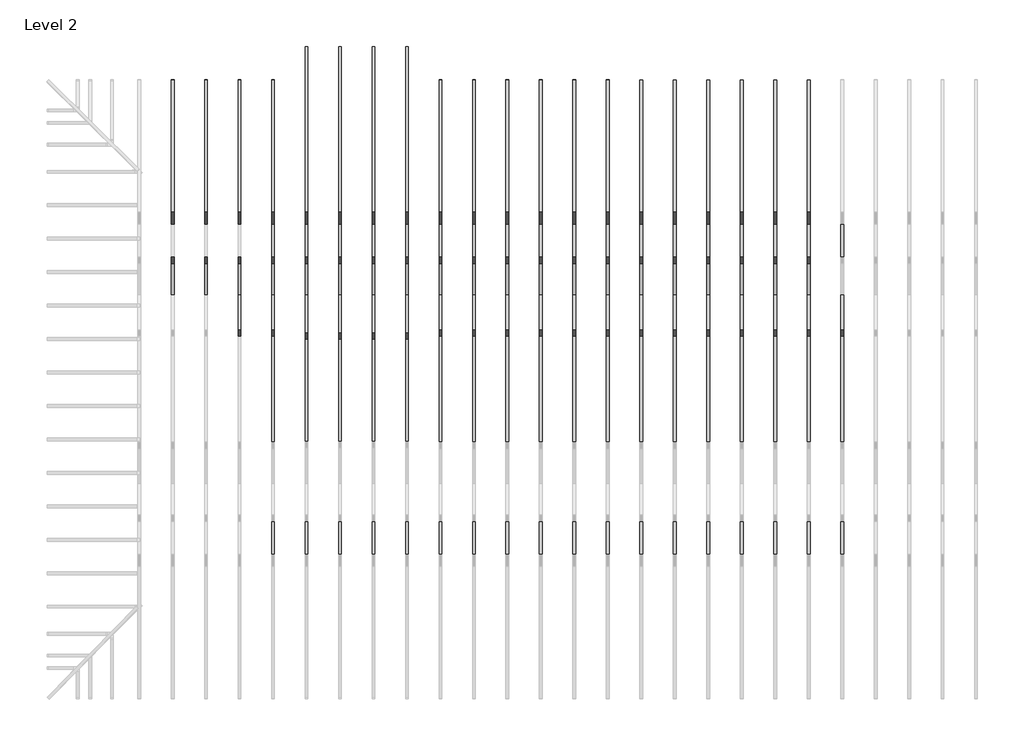
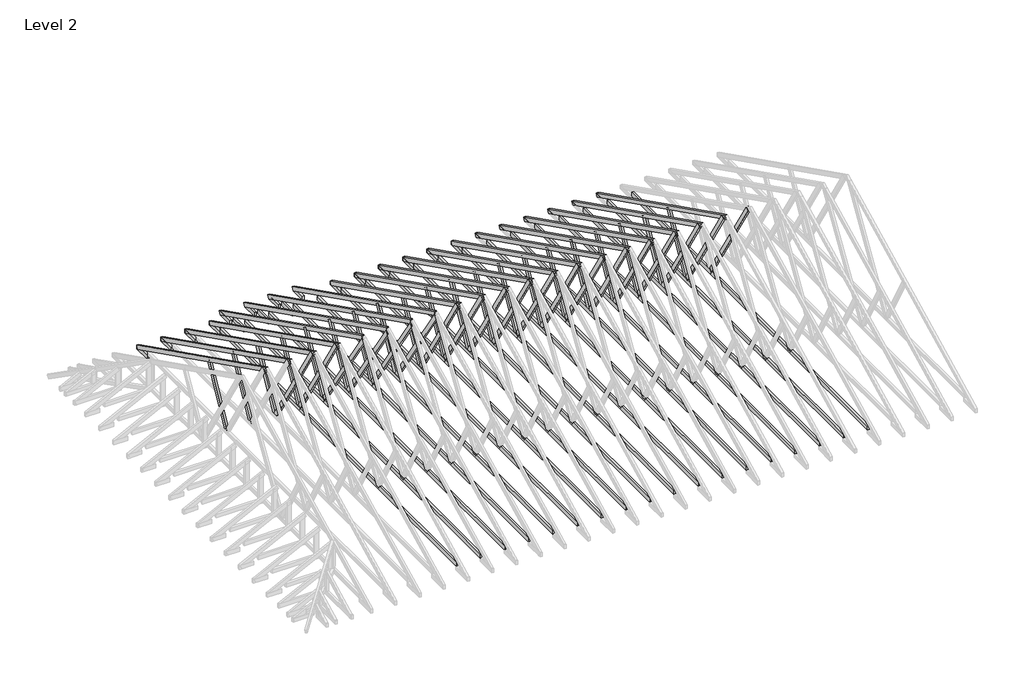
# One storey, part 4 of 5: 96 beams.
"""IFC4 building model written with IfcOpenShell, lengths in millimetres."""

import ifcopenshell
import ifcopenshell.guid

model = None  # the IFC model being written
_history = None  # IfcOwnerHistory: only IFC2X3 demands one
_inside = {}  # id of a spatial element -> (the spatial element, [elements in it])
_under = {}  # id of a project, library or spatial element -> (it, [spatial elements below it])
_declared = {}  # id of a project -> (the project, [libraries it declares])
_typed = {}  # id of a type object -> (the type object, [elements of that type])
_made_of = {}  # id of a material, layer set ... -> (it, [elements and type objects made of it])


def new_model(schema):
    """Start an empty IFC model of exactly this schema.

    Asked for "IFC4X3", IfcOpenShell would pick the latest addendum, in which some entities
    have other attributes; the version numbers below select the first issue.
    IFC2X3 requires an IfcOwnerHistory on every rooted entity: one is made here for all.
    """
    global model, _history
    if schema == "IFC4X3":
        model = ifcopenshell.file(schema_version=(4, 3, 0, 0))
    else:
        model = ifcopenshell.file(schema=schema)
    _inside.clear()
    _under.clear()
    _declared.clear()
    _typed.clear()
    _made_of.clear()
    _history = None
    if model.schema == "IFC2X3":
        org = make("IfcOrganization", Name="unknown")
        user = make(
            "IfcPersonAndOrganization",
            ThePerson=make("IfcPerson", FamilyName="unknown"),
            TheOrganization=org,
        )
        app = make(
            "IfcApplication",
            ApplicationDeveloper=org,
            Version="unknown",
            ApplicationFullName="unknown",
            ApplicationIdentifier="unknown",
        )
        _history = make(
            "IfcOwnerHistory",
            OwningUser=user,
            OwningApplication=app,
            ChangeAction="ADDED",
            CreationDate=0,
        )
    return model


def make(cls, **values):
    """One entity of the class cls with the attributes given. An attribute that is None is left unset."""
    return model.create_entity(
        cls, **{name: value for name, value in values.items() if value is not None}
    )


def rooted(cls, **values):
    """An entity with a GlobalId (a new one), such as an element, a storey or a relation."""
    return make(cls, GlobalId=ifcopenshell.guid.new(), OwnerHistory=_history, **values)


def si_unit(unit_type, name, prefix=None):
    """IfcSIUnit, for example si_unit("LENGTHUNIT", "METRE", prefix="MILLI")."""
    return make("IfcSIUnit", UnitType=unit_type, Prefix=prefix, Name=name)


def assignment(units):
    """IfcUnitAssignment: the units of a project."""
    return None if units is None else make("IfcUnitAssignment", Units=units)


def point(xyz):
    """IfcCartesianPoint."""
    return None if xyz is None else make("IfcCartesianPoint", Coordinates=xyz)


def direction(xyz):
    """IfcDirection."""
    return None if xyz is None else make("IfcDirection", DirectionRatios=xyz)


def frame(location, z_axis=None, x_axis=None):
    """IfcAxis2Placement3D, a coordinate frame: its origin and axes. An axis left out is left unset."""
    return make(
        "IfcAxis2Placement3D",
        Location=point(location),
        Axis=direction(z_axis),
        RefDirection=direction(x_axis),
    )


def origin():
    """The frame at (0, 0, 0) with its axes left unset."""
    return frame((0.0, 0.0, 0.0))


def place(relative_to, where):
    """IfcLocalPlacement: puts the frame where relative to a parent placement (None: the world)."""
    return make(
        "IfcLocalPlacement", PlacementRelTo=relative_to, RelativePlacement=where
    )


def context(
    kind, dimensions, precision=None, world=None, true_north=None, identifier=None
):
    """IfcGeometricRepresentationContext, for example the 3D "Model" context."""
    return make(
        "IfcGeometricRepresentationContext",
        ContextIdentifier=identifier,
        ContextType=kind,
        CoordinateSpaceDimension=dimensions,
        Precision=precision,
        WorldCoordinateSystem=world,
        TrueNorth=true_north,
    )


def project(units=None, contexts=None):
    """IfcProject with its units and contexts."""
    return rooted(
        "IfcProject",
        Name="project",
        RepresentationContexts=contexts,
        UnitsInContext=assignment(units),
    )


def spatial(cls, under=None, at=None, **own):
    """A site, building, storey or space (cls), placed at a placement, below another one or the project."""
    s = rooted(cls, ObjectPlacement=at, **own)
    if under is not None:
        _under.setdefault(under.id(), (under, []))[1].append(s)
    return s


def polyline(points):
    """IfcPolyline through the points."""
    return make("IfcPolyline", Points=[point(p) for p in points])


def outline(outer, holes=None, kind="AREA"):
    """IfcArbitraryClosedProfileDef: a profile drawn as a closed curve; with holes, ...WithVoids."""
    if holes is None:
        return make("IfcArbitraryClosedProfileDef", ProfileType=kind, OuterCurve=outer)
    return make(
        "IfcArbitraryProfileDefWithVoids",
        ProfileType=kind,
        OuterCurve=outer,
        InnerCurves=holes,
    )


def extrude(swept, where, along, depth):
    """IfcExtrudedAreaSolid: the profile swept, set in the frame where, extruded along a direction by depth."""
    return make(
        "IfcExtrudedAreaSolid",
        SweptArea=swept,
        Position=where,
        ExtrudedDirection=direction(along),
        Depth=depth,
    )


def shape(context_of_items, identifier, shape_type, items):
    """IfcShapeRepresentation: the items that make up one representation, for example the "Body"."""
    return make(
        "IfcShapeRepresentation",
        ContextOfItems=context_of_items,
        RepresentationIdentifier=identifier,
        RepresentationType=shape_type,
        Items=items,
    )


def source(mapping_origin, context_of_items, identifier, shape_type, items):
    """IfcRepresentationMap: a shape defined once, which mapped items show again and again."""
    return make(
        "IfcRepresentationMap",
        MappingOrigin=mapping_origin,
        MappedRepresentation=shape(context_of_items, identifier, shape_type, items),
    )


def transform(
    local_origin,
    x_axis=None,
    y_axis=None,
    z_axis=None,
    scale=None,
    scale2=None,
    scale3=None,
    uniform=True,
):
    """IfcCartesianTransformationOperator3D, or its non-uniform kind. x_axis, y_axis, z_axis: its Axis1, 2, 3."""
    if uniform:
        return make(
            "IfcCartesianTransformationOperator3D",
            Axis1=direction(x_axis),
            Axis2=direction(y_axis),
            LocalOrigin=point(local_origin),
            Scale=scale,
            Axis3=direction(z_axis),
        )
    return make(
        "IfcCartesianTransformationOperator3DnonUniform",
        Axis1=direction(x_axis),
        Axis2=direction(y_axis),
        LocalOrigin=point(local_origin),
        Scale=scale,
        Axis3=direction(z_axis),
        Scale2=scale2,
        Scale3=scale3,
    )


def mapped(mapping_source, mapping_target):
    """IfcMappedItem: shows the shape of a source again, moved by a transform."""
    return make(
        "IfcMappedItem", MappingSource=mapping_source, MappingTarget=mapping_target
    )


def made_of(thing, what):
    """Note that an element or type object is made of a material, layer set ...; save() writes the relation."""
    if what is not None:
        _made_of.setdefault(what.id(), (what, []))[1].append(thing)
    return thing


def element(
    cls,
    number,
    at=None,
    inside=None,
    cuts=None,
    type_object=None,
    material=None,
    context=None,
    identifier="Body",
    shape_type=None,
    held_by="IfcProductDefinitionShape",
    body=None,
    shapes=None,
    **own,
):
    """One element of the class cls, such as IfcWall. Its Tag is "e" and its number.

    at: its placement. inside: the storey or other place that contains it. cuts: it is an
    opening in that element (IfcRelVoidsElement). A single representation is given by context,
    identifier, shape_type and body (its items); several are given by shapes. held_by: the class
    of the entity that holds the representations. save() writes the other relations.
    """
    e = rooted(cls, Tag="e%d" % number, ObjectPlacement=at, **own)
    if body is not None:
        shapes = [shape(context, identifier, shape_type, body)]
    if shapes is not None:
        e.Representation = make(held_by, Representations=shapes)
    if inside is not None:
        _inside.setdefault(inside.id(), (inside, []))[1].append(e)
    if cuts is not None:
        rooted(
            "IfcRelVoidsElement", RelatingBuildingElement=cuts, RelatedOpeningElement=e
        )
    if type_object is not None:
        _typed.setdefault(type_object.id(), (type_object, []))[1].append(e)
    return made_of(e, material)


def aggregate(whole, parts):
    """IfcRelAggregates: a whole, such as a stair, and the parts it consists of."""
    return rooted("IfcRelAggregates", RelatingObject=whole, RelatedObjects=parts)


def save(model, path):
    """Write the relations noted so far, then the file.

    IfcRelAggregates (storeys below a building ...), IfcRelContainedInSpatialStructure (elements
    in a storey), IfcRelDefinesByType, IfcRelAssociatesMaterial and IfcRelDeclares: one each for
    every whole, place, type object, material and project.
    """
    for whole, parts in _under.values():
        aggregate(whole, parts)
    for where, things in _inside.values():
        rooted(
            "IfcRelContainedInSpatialStructure",
            RelatedElements=things,
            RelatingStructure=where,
        )
    for kind, things in _typed.values():
        rooted("IfcRelDefinesByType", RelatedObjects=things, RelatingType=kind)
    for what, things in _made_of.values():
        rooted("IfcRelAssociatesMaterial", RelatedObjects=things, RelatingMaterial=what)
    for by, libraries in _declared.values():
        rooted("IfcRelDeclares", RelatingContext=by, RelatedDefinitions=libraries)
    model.write(path)


def beam_b78a0881(model_context):
    return source(origin(), model_context, "Body", "SweptSolid", [
        extrude(outline(polyline([(228.6, 25.4), (228.6, -25.4), (-228.6, -25.4), (-228.6, 25.4), (228.6, 25.4)])), frame((0.0, 0.0, -50.8), z_axis=(0.0, 0.0, 1.0), x_axis=(1.0, 0.0, 0.0)), (0.0, 0.0, 1.0), 101.6),
    ])


def beam_90eea034(model_context):
    return source(origin(), model_context, "Body", "SweptSolid", [
        extrude(outline(polyline([(821.193698, 25.4), (821.193698, -25.4), (-819.5010489, -25.4), (-819.5010489, 25.4), (821.193698, 25.4)])), frame((0.0, 0.0, -50.8), z_axis=(0.0, 0.0, 1.0), x_axis=(1.0, 0.0, 0.0)), (0.0, 0.0, 1.0), 101.6),
    ])


def beam_a4242642(model_context):
    return source(origin(), model_context, "Body", "SweptSolid", [
        extrude(outline(polyline([(5145.3336481, 25.4), (5145.3336481, -25.4), (-5145.3336481, -25.4), (-5145.3336481, 25.4), (5145.3336481, 25.4)])), frame((0.0, 0.0, -50.8), z_axis=(0.0, 0.0, 1.0), x_axis=(1.0, 0.0, 0.0)), (0.0, 0.0, 1.0), 101.6),
    ])


def beam_fc8bf4ae(model_context):
    return source(origin(), model_context, "Body", "SweptSolid", [
        extrude(outline(polyline([(1562.6646551, 25.4), (1562.6646551, -25.4), (-1550.1468127, -25.4), (-1550.1468127, 25.4), (1562.6646551, 25.4)])), frame((0.0, 0.0, -50.8), z_axis=(0.0, 0.0, 1.0), x_axis=(1.0, 0.0, 0.0)), (0.0, 0.0, 1.0), 101.6),
    ])


def beam_2924e986(model_context):
    return source(origin(), model_context, "Body", "SweptSolid", [
        extrude(outline(polyline([(228.5999994, 25.4), (228.5999994, -25.4), (-179.8629717, -25.4), (-179.8629717, 25.4), (228.5999994, 25.4)])), frame((0.0, 0.0, -50.8), z_axis=(0.0, 0.0, 1.0), x_axis=(1.0, 0.0, 0.0)), (0.0, 0.0, 1.0), 101.6),
    ])


def beam_189f326c(model_context):
    return source(origin(), model_context, "Body", "SweptSolid", [
        extrude(outline(polyline([(1574.4380265, 25.4), (1574.4380265, -25.4), (-1601.4606477, -25.4), (-1601.4606477, 25.4), (1574.4380265, 25.4)])), frame((0.0, 0.0, -50.8), z_axis=(0.0, 0.0, 1.0), x_axis=(1.0, 0.0, 0.0)), (0.0, 0.0, 1.0), 101.6),
    ])


def beam_af7bd0b6(model_context):
    return source(origin(), model_context, "Body", "SweptSolid", [
        extrude(outline(polyline([(228.6, 25.4), (228.6, -25.4), (-179.8629717, -25.4), (-179.8629717, 25.4), (228.6, 25.4)])), frame((0.0, 0.0, -50.8), z_axis=(0.0, 0.0, 1.0), x_axis=(1.0, 0.0, 0.0)), (0.0, 0.0, 1.0), 101.6),
    ])


model = new_model("IFC4")

# Units and contexts
model_context = context("Model", 3, world=origin())
ifc_project = project(units=[si_unit("LENGTHUNIT", "METRE", prefix="MILLI")], contexts=[model_context])

# Site, building, storey
site = spatial("IfcSite", under=ifc_project)
building = spatial("IfcBuilding", under=site)
storey = spatial("IfcBuildingStorey", under=building, Name="Level 2", Elevation=2768.6)

# Beams
placement = place(None, origin())
element("IfcBeam", 1, ObjectType="Dimension Lumber : BLDG 6241 2X4\" TRUSS MEMBER", at=placement, inside=storey, context=model_context, shape_type="SweptSolid", body=[
    extrude(outline(polyline([(0.0, -50.8), (0.0, 0.0), (6948.260151, 0.0), (6948.260151, -50.8), (0.0, -50.8)])), frame((-13559.414829, 10.7781069, 5482.082899), z_axis=(0.0, 0.4472135954999579, 0.894427190999916), x_axis=(0.0, 0.894427190999916, -0.4472135954999579)), (0.0, 0.0, 1.0), 101.6),
])
element("IfcBeam", 2, ObjectType="Dimension Lumber : BLDG 6241 2X4\" TRUSS MEMBER", at=placement, inside=storey, context=model_context, shape_type="SweptSolid", body=[
    extrude(outline(polyline([(0.0, -50.8), (0.0, 0.0), (6948.260151, 0.0), (6948.260151, -50.8), (0.0, -50.8)])), frame((-12949.814829, 10.7781069, 5482.082899), z_axis=(0.0, 0.44721359549995804, 0.894427190999916), x_axis=(0.0, 0.894427190999916, -0.44721359549995804)), (0.0, 0.0, 1.0), 101.6),
])
element("IfcBeam", 3, ObjectType="Dimension Lumber : BLDG 6241 2X4\" TRUSS MEMBER", at=placement, inside=storey, context=model_context, shape_type="SweptSolid", body=[
    extrude(outline(polyline([(0.0, -50.8), (0.0, 0.0), (6948.260151, 0.0), (6948.260151, -50.8), (0.0, -50.8)])), frame((-12340.214829, 10.7781069, 5482.082899), z_axis=(0.0, 0.44721359549995804, 0.894427190999916), x_axis=(0.0, 0.894427190999916, -0.44721359549995804)), (0.0, 0.0, 1.0), 101.6),
])
element("IfcBeam", 4, ObjectType="Dimension Lumber : BLDG 6241 2X4\" TRUSS MEMBER", at=placement, inside=storey, context=model_context, shape_type="SweptSolid", body=[
    extrude(outline(polyline([(0.0, -50.8), (0.0, 0.0), (6948.260151, 0.0), (6948.260151, -50.8), (0.0, -50.8)])), frame((-11730.614829, 10.7781069, 5482.082899), z_axis=(0.0, 0.44721359549995804, 0.894427190999916), x_axis=(0.0, 0.894427190999916, -0.44721359549995804)), (0.0, 0.0, 1.0), 101.6),
])
element("IfcBeam", 5, ObjectType="Dimension Lumber : BLDG 6241 2X4\" TRUSS MEMBER", at=placement, inside=storey, context=model_context, shape_type="SweptSolid", body=[
    extrude(outline(polyline([(0.0, -50.8), (0.0, 0.0), (6302.2496334, 0.0), (6302.2496334, -50.8), (0.0, -50.8)])), frame((-15997.814829, -17.2791662, 5496.1115355), z_axis=(0.0, 0.447213595499956, 0.894427190999917), x_axis=(0.0, 0.894427190999917, -0.447213595499956)), (0.0, 0.0, 1.0), 101.6),
])
element("IfcBeam", 6, ObjectType="Dimension Lumber : BLDG 6241 2X4\" TRUSS MEMBER", at=placement, inside=storey, context=model_context, shape_type="SweptSolid", body=[
    extrude(outline(polyline([(0.0, -50.8), (0.0, 0.0), (6302.2496334, 0.0), (6302.2496334, -50.8), (0.0, -50.8)])), frame((-15388.214829, -17.2791662, 5496.1115355), z_axis=(0.0, 0.447213595499956, 0.894427190999917), x_axis=(0.0, 0.894427190999917, -0.447213595499956)), (0.0, 0.0, 1.0), 101.6),
])
element("IfcBeam", 7, ObjectType="Dimension Lumber : BLDG 6241 2X4\" TRUSS MEMBER", at=placement, inside=storey, context=model_context, shape_type="SweptSolid", body=[
    extrude(outline(polyline([(0.0, -50.8), (0.0, 0.0), (6302.2496334, 0.0), (6302.2496334, -50.8), (0.0, -50.8)])), frame((-14778.614829, -17.2791662, 5496.1115355), z_axis=(0.0, 0.44721359549995576, 0.8944271909999171), x_axis=(0.0, 0.8944271909999171, -0.44721359549995576)), (0.0, 0.0, 1.0), 101.6),
])
element("IfcBeam", 8, ObjectType="Dimension Lumber : BLDG 6241 2X4\" TRUSS MEMBER", at=placement, inside=storey, context=model_context, shape_type="SweptSolid", body=[
    extrude(outline(polyline([(0.0, -50.8), (0.0, 0.0), (6302.2496334, 0.0), (6302.2496334, -50.8), (0.0, -50.8)])), frame((-14169.014829, -17.2791662, 5496.1115355), z_axis=(0.0, 0.447213595499956, 0.894427190999917), x_axis=(0.0, 0.894427190999917, -0.447213595499956)), (0.0, 0.0, 1.0), 101.6),
])
element("IfcBeam", 9, ObjectType="Dimension Lumber : BLDG 6241 2X4\" TRUSS MEMBER", at=placement, inside=storey, context=model_context, shape_type="SweptSolid", body=[
    extrude(outline(polyline([(0.0, -50.8), (0.0, 0.0), (6302.2496334, 0.0), (6302.2496334, -50.8), (0.0, -50.8)])), frame((-11121.014829, -17.2791662, 5496.1115355), z_axis=(0.0, 0.447213595499956, 0.894427190999917), x_axis=(0.0, 0.894427190999917, -0.447213595499956)), (0.0, 0.0, 1.0), 101.6),
])
element("IfcBeam", 10, ObjectType="Dimension Lumber : BLDG 6241 2X4\" TRUSS MEMBER", at=placement, inside=storey, context=model_context, shape_type="SweptSolid", body=[
    extrude(outline(polyline([(0.0, -50.8), (0.0, 0.0), (6302.2496334, 0.0), (6302.2496334, -50.8), (0.0, -50.8)])), frame((-10511.414829, -17.2791662, 5496.1115355), z_axis=(0.0, 0.4472135954999559, 0.894427190999917), x_axis=(0.0, 0.894427190999917, -0.4472135954999559)), (0.0, 0.0, 1.0), 101.6),
])
element("IfcBeam", 11, ObjectType="Dimension Lumber : BLDG 6241 2X4\" TRUSS MEMBER", at=placement, inside=storey, context=model_context, shape_type="SweptSolid", body=[
    extrude(outline(polyline([(0.0, -50.8), (0.0, 0.0), (6302.2496334, 0.0), (6302.2496334, -50.8), (0.0, -50.8)])), frame((-9901.814829, -17.2791662, 5496.1115355), z_axis=(0.0, 0.44721359549995576, 0.894427190999917), x_axis=(0.0, 0.894427190999917, -0.44721359549995576)), (0.0, 0.0, 1.0), 101.6),
])
element("IfcBeam", 12, ObjectType="Dimension Lumber : BLDG 6241 2X4\" TRUSS MEMBER", at=placement, inside=storey, context=model_context, shape_type="SweptSolid", body=[
    extrude(outline(polyline([(0.0, -50.8), (0.0, 0.0), (6302.2496334, 0.0), (6302.2496334, -50.8), (0.0, -50.8)])), frame((-9292.214829, -17.2791662, 5496.1115355), z_axis=(0.0, 0.447213595499956, 0.8944271909999169), x_axis=(0.0, 0.8944271909999169, -0.447213595499956)), (0.0, 0.0, 1.0), 101.6),
])
element("IfcBeam", 13, ObjectType="Dimension Lumber : BLDG 6241 2X4\" TRUSS MEMBER", at=placement, inside=storey, context=model_context, shape_type="SweptSolid", body=[
    extrude(outline(polyline([(0.0, -50.8), (0.0, 0.0), (6302.2496334, 0.0), (6302.2496334, -50.8), (0.0, -50.8)])), frame((-8682.614829, -17.2791662, 5496.1115355), z_axis=(0.0, 0.44721359549995593, 0.894427190999917), x_axis=(0.0, 0.894427190999917, -0.44721359549995593)), (0.0, 0.0, 1.0), 101.6),
])
element("IfcBeam", 14, ObjectType="Dimension Lumber : BLDG 6241 2X4\" TRUSS MEMBER", at=placement, inside=storey, context=model_context, shape_type="SweptSolid", body=[
    extrude(outline(polyline([(0.0, -50.8), (0.0, 0.0), (6302.2496334, 0.0), (6302.2496334, -50.8), (0.0, -50.8)])), frame((-8073.014829, -17.2791662, 5496.1115355), z_axis=(0.0, 0.4472135954999558, 0.894427190999917), x_axis=(0.0, 0.894427190999917, -0.4472135954999558)), (0.0, 0.0, 1.0), 101.6),
])
element("IfcBeam", 15, ObjectType="Dimension Lumber : BLDG 6241 2X4\" TRUSS MEMBER", at=placement, inside=storey, context=model_context, shape_type="SweptSolid", body=[
    extrude(outline(polyline([(0.0, -50.8), (0.0, 0.0), (6302.2496334, 0.0), (6302.2496334, -50.8), (0.0, -50.8)])), frame((-7463.414829, -17.2791662, 5496.1115355), z_axis=(0.0, 0.4472135954999557, 0.894427190999917), x_axis=(0.0, 0.894427190999917, -0.4472135954999557)), (0.0, 0.0, 1.0), 101.6),
])
element("IfcBeam", 16, ObjectType="Dimension Lumber : BLDG 6241 2X4\" TRUSS MEMBER", at=placement, inside=storey, context=model_context, shape_type="SweptSolid", body=[
    extrude(outline(polyline([(0.0, -50.8), (0.0, 0.0), (6302.2496334, 0.0), (6302.2496334, -50.8), (0.0, -50.8)])), frame((-6853.814829, -17.2791662, 5496.1115355), z_axis=(0.0, 0.4472135954999561, 0.8944271909999169), x_axis=(0.0, 0.8944271909999169, -0.4472135954999561)), (0.0, 0.0, 1.0), 101.6),
])
element("IfcBeam", 17, ObjectType="Dimension Lumber : BLDG 6241 2X4\" TRUSS MEMBER", at=placement, inside=storey, context=model_context, shape_type="SweptSolid", body=[
    extrude(outline(polyline([(0.0, -50.8), (0.0, 0.0), (6302.2496334, 0.0), (6302.2496334, -50.8), (0.0, -50.8)])), frame((-6244.214829, -17.2791662, 5496.1115355), z_axis=(0.0, 0.44721359549995593, 0.894427190999917), x_axis=(0.0, 0.894427190999917, -0.44721359549995593)), (0.0, 0.0, 1.0), 101.6),
])
element("IfcBeam", 18, ObjectType="Dimension Lumber : BLDG 6241 2X4\" TRUSS MEMBER", at=placement, inside=storey, context=model_context, shape_type="SweptSolid", body=[
    extrude(outline(polyline([(0.0, -50.8), (0.0, 0.0), (6302.2496334, 0.0), (6302.2496334, -50.8), (0.0, -50.8)])), frame((-5634.614829, -17.2791662, 5496.1115355), z_axis=(0.0, 0.447213595499956, 0.8944271909999169), x_axis=(0.0, 0.8944271909999169, -0.447213595499956)), (0.0, 0.0, 1.0), 101.6),
])
element("IfcBeam", 19, ObjectType="Dimension Lumber : BLDG 6241 2X4\" TRUSS MEMBER", at=placement, inside=storey, context=model_context, shape_type="SweptSolid", body=[
    extrude(outline(polyline([(0.0, -50.8), (0.0, 0.0), (6302.2496334, 0.0), (6302.2496334, -50.8), (0.0, -50.8)])), frame((-5025.014829, -17.2791662, 5496.1115355), z_axis=(0.0, 0.44721359549995593, 0.894427190999917), x_axis=(0.0, 0.894427190999917, -0.44721359549995593)), (0.0, 0.0, 1.0), 101.6),
])
element("IfcBeam", 20, ObjectType="Dimension Lumber : BLDG 6241 2X4\" TRUSS MEMBER", at=placement, inside=storey, context=model_context, shape_type="SweptSolid", body=[
    extrude(outline(polyline([(0.0, -50.8), (0.0, 0.0), (6302.2496334, 0.0), (6302.2496334, -50.8), (0.0, -50.8)])), frame((-4415.414829, -17.2791662, 5496.1115355), z_axis=(0.0, 0.4472135954999558, 0.894427190999917), x_axis=(0.0, 0.894427190999917, -0.4472135954999558)), (0.0, 0.0, 1.0), 101.6),
])
beam_shape = beam_b78a0881(model_context)
element("IfcBeam", 21, ObjectType="Dimension Lumber : BLDG 6241 2X4\" TRUSS MEMBER", at=placement, inside=storey, context=model_context, shape_type="MappedRepresentation", body=[
    mapped(beam_shape, transform((-13534.014829, 5436.3284114, 2589.5072623), x_axis=(0.0, -1.0, 0.0), y_axis=(1.0, 0.0, 0.0), z_axis=(0.0, 0.0, 1.0))),
])
element("IfcBeam", 22, ObjectType="Dimension Lumber : BLDG 6241 2X4\" TRUSS MEMBER", at=placement, inside=storey, context=model_context, shape_type="MappedRepresentation", body=[
    mapped(beam_shape, transform((-12924.414829, 5436.3284114, 2589.5072623), x_axis=(0.0, -1.0, 0.0), y_axis=(1.0, 0.0, 0.0), z_axis=(0.0, 0.0, 1.0))),
])
element("IfcBeam", 23, ObjectType="Dimension Lumber : BLDG 6241 2X4\" TRUSS MEMBER", at=placement, inside=storey, context=model_context, shape_type="MappedRepresentation", body=[
    mapped(beam_shape, transform((-12314.814829, 5436.3284114, 2589.5072623), x_axis=(0.0, -1.0, 0.0), y_axis=(1.0, 0.0, 0.0), z_axis=(0.0, 0.0, 1.0))),
])
element("IfcBeam", 24, ObjectType="Dimension Lumber : BLDG 6241 2X4\" TRUSS MEMBER", at=placement, inside=storey, context=model_context, shape_type="MappedRepresentation", body=[
    mapped(beam_shape, transform((-12924.414829, 5436.3284114, 2589.5072623), x_axis=(0.0, -1.0, 0.0), y_axis=(1.0, 0.0, 0.0), z_axis=(0.0, 0.0, 1.0))),
])
element("IfcBeam", 25, ObjectType="Dimension Lumber : BLDG 6241 2X4\" TRUSS MEMBER", at=placement, inside=storey, context=model_context, shape_type="MappedRepresentation", body=[
    mapped(beam_shape, transform((-12314.814829, 5436.3284114, 2589.5072623), x_axis=(0.0, -1.0, 0.0), y_axis=(1.0, 0.0, 0.0), z_axis=(0.0, 0.0, 1.0))),
])
element("IfcBeam", 26, ObjectType="Dimension Lumber : BLDG 6241 2X4\" TRUSS MEMBER", at=placement, inside=storey, context=model_context, shape_type="MappedRepresentation", body=[
    mapped(beam_shape, transform((-15972.414829, 5436.3284114, 2717.8), x_axis=(0.0, -1.0, 0.0), y_axis=(1.0, 0.0, 0.0), z_axis=(0.0, 0.0, 1.0))),
])
element("IfcBeam", 27, ObjectType="Dimension Lumber : BLDG 6241 2X4\" TRUSS MEMBER", at=placement, inside=storey, context=model_context, shape_type="MappedRepresentation", body=[
    mapped(beam_shape, transform((-15362.814829, 5436.3284114, 2717.8), x_axis=(0.0, -1.0, 0.0), y_axis=(1.0, 0.0, 0.0), z_axis=(0.0, 0.0, 1.0))),
])
element("IfcBeam", 28, ObjectType="Dimension Lumber : BLDG 6241 2X4\" TRUSS MEMBER", at=placement, inside=storey, context=model_context, shape_type="MappedRepresentation", body=[
    mapped(beam_shape, transform((-14753.214829, 5436.3284114, 2717.8), x_axis=(0.0, -1.0, 0.0), y_axis=(1.0, 0.0, 0.0), z_axis=(0.0, 0.0, 1.0))),
])
element("IfcBeam", 29, ObjectType="Dimension Lumber : BLDG 6241 2X4\" TRUSS MEMBER", at=placement, inside=storey, context=model_context, shape_type="MappedRepresentation", body=[
    mapped(beam_shape, transform((-14143.614829, 5436.3284114, 2717.8), x_axis=(0.0, -1.0, 0.0), y_axis=(1.0, 0.0, 0.0), z_axis=(0.0, 0.0, 1.0))),
])
element("IfcBeam", 30, ObjectType="Dimension Lumber : BLDG 6241 2X4\" TRUSS MEMBER", at=placement, inside=storey, context=model_context, shape_type="MappedRepresentation", body=[
    mapped(beam_shape, transform((-11095.614829, 5436.3284114, 2717.8), x_axis=(0.0, -1.0, 0.0), y_axis=(1.0, 0.0, 0.0), z_axis=(0.0, 0.0, 1.0))),
])
element("IfcBeam", 31, ObjectType="Dimension Lumber : BLDG 6241 2X4\" TRUSS MEMBER", at=placement, inside=storey, context=model_context, shape_type="MappedRepresentation", body=[
    mapped(beam_shape, transform((-10486.014829, 5436.3284114, 2717.8), x_axis=(0.0, -1.0, 0.0), y_axis=(1.0, 0.0, 0.0), z_axis=(0.0, 0.0, 1.0))),
])
element("IfcBeam", 32, ObjectType="Dimension Lumber : BLDG 6241 2X4\" TRUSS MEMBER", at=placement, inside=storey, context=model_context, shape_type="MappedRepresentation", body=[
    mapped(beam_shape, transform((-9876.414829, 5436.3284114, 2717.8), x_axis=(0.0, -1.0, 0.0), y_axis=(1.0, 0.0, 0.0), z_axis=(0.0, 0.0, 1.0))),
])
element("IfcBeam", 33, ObjectType="Dimension Lumber : BLDG 6241 2X4\" TRUSS MEMBER", at=placement, inside=storey, context=model_context, shape_type="MappedRepresentation", body=[
    mapped(beam_shape, transform((-9266.814829, 5436.3284114, 2717.8), x_axis=(0.0, -1.0, 0.0), y_axis=(1.0, 0.0, 0.0), z_axis=(0.0, 0.0, 1.0))),
])
element("IfcBeam", 34, ObjectType="Dimension Lumber : BLDG 6241 2X4\" TRUSS MEMBER", at=placement, inside=storey, context=model_context, shape_type="MappedRepresentation", body=[
    mapped(beam_shape, transform((-8657.214829, 5436.3284114, 2717.8), x_axis=(0.0, -1.0, 0.0), y_axis=(1.0, 0.0, 0.0), z_axis=(0.0, 0.0, 1.0))),
])
element("IfcBeam", 35, ObjectType="Dimension Lumber : BLDG 6241 2X4\" TRUSS MEMBER", at=placement, inside=storey, context=model_context, shape_type="MappedRepresentation", body=[
    mapped(beam_shape, transform((-8047.614829, 5436.3284114, 2717.8), x_axis=(0.0, -1.0, 0.0), y_axis=(1.0, 0.0, 0.0), z_axis=(0.0, 0.0, 1.0))),
])
beam_2_shape = beam_90eea034(model_context)
element("IfcBeam", 36, ObjectType="Dimension Lumber : BLDG 6241 2X4\" TRUSS MEMBER", at=placement, inside=storey, context=model_context, shape_type="MappedRepresentation", body=[
    mapped(beam_2_shape, transform((-13534.014829, 2147.8781861, 3552.5770493), x_axis=(0.0, -0.48031726308520883, -0.87709482200178), y_axis=(-1.0, 0.0, 0.0), z_axis=(0.0, 0.87709482200178, -0.48031726308520883))),
])
element("IfcBeam", 37, ObjectType="Dimension Lumber : BLDG 6241 2X4\" TRUSS MEMBER", at=placement, inside=storey, context=model_context, shape_type="MappedRepresentation", body=[
    mapped(beam_2_shape, transform((-12924.414829, 2147.8781861, 3552.5770493), x_axis=(0.0, -0.48031726308520883, -0.87709482200178), y_axis=(-1.0, 0.0, 0.0), z_axis=(0.0, 0.87709482200178, -0.48031726308520883))),
])
element("IfcBeam", 38, ObjectType="Dimension Lumber : BLDG 6241 2X4\" TRUSS MEMBER", at=placement, inside=storey, context=model_context, shape_type="MappedRepresentation", body=[
    mapped(beam_2_shape, transform((-12314.814829, 2147.8781861, 3552.5770493), x_axis=(0.0, -0.48031726308520883, -0.87709482200178), y_axis=(-1.0, 0.0, 0.0), z_axis=(0.0, 0.87709482200178, -0.48031726308520883))),
])
element("IfcBeam", 39, ObjectType="Dimension Lumber : BLDG 6241 2X4\" TRUSS MEMBER", at=placement, inside=storey, context=model_context, shape_type="MappedRepresentation", body=[
    mapped(beam_2_shape, transform((-11705.214829, 2147.8781861, 3552.5770493), x_axis=(0.0, -0.48031726308520883, -0.87709482200178), y_axis=(-1.0, 0.0, 0.0), z_axis=(0.0, 0.87709482200178, -0.48031726308520883))),
])
element("IfcBeam", 40, ObjectType="Dimension Lumber : BLDG 6241 2X4\" TRUSS MEMBER", at=placement, inside=storey, context=model_context, shape_type="MappedRepresentation", body=[
    mapped(beam_2_shape, transform((-15972.414829, 2147.8781861, 3552.5770493), x_axis=(0.0, -0.4803172630852004, -0.8770948220017847), y_axis=(-1.0, 0.0, 0.0), z_axis=(0.0, 0.8770948220017847, -0.4803172630852004))),
])
element("IfcBeam", 41, ObjectType="Dimension Lumber : BLDG 6241 2X4\" TRUSS MEMBER", at=placement, inside=storey, context=model_context, shape_type="MappedRepresentation", body=[
    mapped(beam_2_shape, transform((-15362.814829, 2147.8781861, 3552.5770493), x_axis=(0.0, -0.4803172630852004, -0.8770948220017847), y_axis=(-1.0, 0.0, 0.0), z_axis=(0.0, 0.8770948220017847, -0.4803172630852004))),
])
element("IfcBeam", 42, ObjectType="Dimension Lumber : BLDG 6241 2X4\" TRUSS MEMBER", at=placement, inside=storey, context=model_context, shape_type="MappedRepresentation", body=[
    mapped(beam_2_shape, transform((-14753.214829, 2147.8781861, 3552.5770493), x_axis=(0.0, -0.4803172630852004, -0.8770948220017847), y_axis=(-1.0, 0.0, 0.0), z_axis=(0.0, 0.8770948220017847, -0.4803172630852004))),
])
element("IfcBeam", 43, ObjectType="Dimension Lumber : BLDG 6241 2X4\" TRUSS MEMBER", at=placement, inside=storey, context=model_context, shape_type="MappedRepresentation", body=[
    mapped(beam_2_shape, transform((-14143.614829, 2147.8781861, 3552.5770493), x_axis=(0.0, -0.4803172630852004, -0.8770948220017847), y_axis=(-1.0, 0.0, 0.0), z_axis=(0.0, 0.8770948220017847, -0.4803172630852004))),
])
element("IfcBeam", 44, ObjectType="Dimension Lumber : BLDG 6241 2X4\" TRUSS MEMBER", at=placement, inside=storey, context=model_context, shape_type="MappedRepresentation", body=[
    mapped(beam_2_shape, transform((-11095.614829, 2147.8781861, 3552.5770493), x_axis=(0.0, -0.4803172630852004, -0.8770948220017847), y_axis=(-1.0, 0.0, 0.0), z_axis=(0.0, 0.8770948220017847, -0.4803172630852004))),
])
element("IfcBeam", 45, ObjectType="Dimension Lumber : BLDG 6241 2X4\" TRUSS MEMBER", at=placement, inside=storey, context=model_context, shape_type="MappedRepresentation", body=[
    mapped(beam_2_shape, transform((-10486.014829, 2147.8781861, 3552.5770493), x_axis=(0.0, -0.4803172630852004, -0.8770948220017847), y_axis=(-1.0, 0.0, 0.0), z_axis=(0.0, 0.8770948220017847, -0.4803172630852004))),
])
element("IfcBeam", 46, ObjectType="Dimension Lumber : BLDG 6241 2X4\" TRUSS MEMBER", at=placement, inside=storey, context=model_context, shape_type="MappedRepresentation", body=[
    mapped(beam_2_shape, transform((-9876.414829, 2147.8781861, 3552.5770493), x_axis=(0.0, -0.4803172630852004, -0.8770948220017847), y_axis=(-1.0, 0.0, 0.0), z_axis=(0.0, 0.8770948220017847, -0.4803172630852004))),
])
element("IfcBeam", 47, ObjectType="Dimension Lumber : BLDG 6241 2X4\" TRUSS MEMBER", at=placement, inside=storey, context=model_context, shape_type="MappedRepresentation", body=[
    mapped(beam_2_shape, transform((-9266.814829, 2147.8781861, 3552.5770493), x_axis=(0.0, -0.4803172630852004, -0.8770948220017847), y_axis=(-1.0, 0.0, 0.0), z_axis=(0.0, 0.8770948220017847, -0.4803172630852004))),
])
element("IfcBeam", 48, ObjectType="Dimension Lumber : BLDG 6241 2X4\" TRUSS MEMBER", at=placement, inside=storey, context=model_context, shape_type="MappedRepresentation", body=[
    mapped(beam_2_shape, transform((-8657.214829, 2147.8781861, 3552.5770493), x_axis=(0.0, -0.4803172630852004, -0.8770948220017847), y_axis=(-1.0, 0.0, 0.0), z_axis=(0.0, 0.8770948220017847, -0.4803172630852004))),
])
element("IfcBeam", 49, ObjectType="Dimension Lumber : BLDG 6241 2X4\" TRUSS MEMBER", at=placement, inside=storey, context=model_context, shape_type="MappedRepresentation", body=[
    mapped(beam_2_shape, transform((-8047.614829, 2147.8781861, 3552.5770493), x_axis=(0.0, -0.4803172630852004, -0.8770948220017847), y_axis=(-1.0, 0.0, 0.0), z_axis=(0.0, 0.8770948220017847, -0.4803172630852004))),
])
element("IfcBeam", 50, ObjectType="Dimension Lumber : BLDG 6241 2X4\" TRUSS MEMBER", at=placement, inside=storey, context=model_context, shape_type="MappedRepresentation", body=[
    mapped(beam_2_shape, transform((-7438.014829, 2147.8781861, 3552.5770493), x_axis=(0.0, -0.4803172630852004, -0.8770948220017847), y_axis=(-1.0, 0.0, 0.0), z_axis=(0.0, 0.8770948220017847, -0.4803172630852004))),
])
element("IfcBeam", 51, ObjectType="Dimension Lumber : BLDG 6241 2X4\" TRUSS MEMBER", at=placement, inside=storey, context=model_context, shape_type="MappedRepresentation", body=[
    mapped(beam_2_shape, transform((-6828.414829, 2147.8781861, 3552.5770493), x_axis=(0.0, -0.4803172630852004, -0.8770948220017847), y_axis=(-1.0, 0.0, 0.0), z_axis=(0.0, 0.8770948220017847, -0.4803172630852004))),
])
element("IfcBeam", 52, ObjectType="Dimension Lumber : BLDG 6241 2X4\" TRUSS MEMBER", at=placement, inside=storey, context=model_context, shape_type="MappedRepresentation", body=[
    mapped(beam_2_shape, transform((-6218.814829, 2147.8781861, 3552.5770493), x_axis=(0.0, -0.4803172630852004, -0.8770948220017847), y_axis=(-1.0, 0.0, 0.0), z_axis=(0.0, 0.8770948220017847, -0.4803172630852004))),
])
element("IfcBeam", 53, ObjectType="Dimension Lumber : BLDG 6241 2X4\" TRUSS MEMBER", at=placement, inside=storey, context=model_context, shape_type="MappedRepresentation", body=[
    mapped(beam_2_shape, transform((-5609.214829, 2147.8781861, 3552.5770493), x_axis=(0.0, -0.4803172630852004, -0.8770948220017847), y_axis=(-1.0, 0.0, 0.0), z_axis=(0.0, 0.8770948220017847, -0.4803172630852004))),
])
element("IfcBeam", 54, ObjectType="Dimension Lumber : BLDG 6241 2X4\" TRUSS MEMBER", at=placement, inside=storey, context=model_context, shape_type="MappedRepresentation", body=[
    mapped(beam_2_shape, transform((-4999.614829, 2147.8781861, 3552.5770493), x_axis=(0.0, -0.4803172630852004, -0.8770948220017847), y_axis=(-1.0, 0.0, 0.0), z_axis=(0.0, 0.8770948220017847, -0.4803172630852004))),
])
element("IfcBeam", 55, ObjectType="Dimension Lumber : BLDG 6241 2X4\" TRUSS MEMBER", at=placement, inside=storey, context=model_context, shape_type="MappedRepresentation", body=[
    mapped(beam_2_shape, transform((-4390.014829, 2147.8781861, 3552.5770493), x_axis=(0.0, -0.4803172630852004, -0.8770948220017847), y_axis=(-1.0, 0.0, 0.0), z_axis=(0.0, 0.8770948220017847, -0.4803172630852004))),
])
beam_3_shape = beam_a4242642(model_context)
element("IfcBeam", 56, ObjectType="Dimension Lumber : BLDG 6241 2X4\" TRUSS MEMBER", at=placement, inside=storey, context=model_context, shape_type="MappedRepresentation", body=[
    mapped(beam_3_shape, transform((-13534.014829, 26.1284114, 2819.4), x_axis=(0.0, -1.0, 0.0), y_axis=(1.0, 0.0, 0.0), z_axis=(0.0, 0.0, 1.0))),
])
element("IfcBeam", 57, ObjectType="Dimension Lumber : BLDG 6241 2X4\" TRUSS MEMBER", at=placement, inside=storey, context=model_context, shape_type="MappedRepresentation", body=[
    mapped(beam_3_shape, transform((-12924.414829, 26.1284114, 2819.4), x_axis=(0.0, -1.0, 0.0), y_axis=(1.0, 0.0, 0.0), z_axis=(0.0, 0.0, 1.0))),
])
element("IfcBeam", 58, ObjectType="Dimension Lumber : BLDG 6241 2X4\" TRUSS MEMBER", at=placement, inside=storey, context=model_context, shape_type="MappedRepresentation", body=[
    mapped(beam_3_shape, transform((-12314.814829, 26.1284114, 2819.4), x_axis=(0.0, -1.0, 0.0), y_axis=(1.0, 0.0, 0.0), z_axis=(0.0, 0.0, 1.0))),
])
element("IfcBeam", 59, ObjectType="Dimension Lumber : BLDG 6241 2X4\" TRUSS MEMBER", at=placement, inside=storey, context=model_context, shape_type="MappedRepresentation", body=[
    mapped(beam_3_shape, transform((-11705.214829, 26.1284114, 2819.4), x_axis=(0.0, -1.0, 0.0), y_axis=(1.0, 0.0, 0.0), z_axis=(0.0, 0.0, 1.0))),
])
element("IfcBeam", 60, ObjectType="Dimension Lumber : BLDG 6241 2X4\" TRUSS MEMBER", at=placement, inside=storey, context=model_context, shape_type="MappedRepresentation", body=[
    mapped(beam_3_shape, transform((-14143.614829, 26.1284114, 2819.4), x_axis=(0.0, -1.0, 0.0), y_axis=(1.0, 0.0, 0.0), z_axis=(0.0, 0.0, 1.0))),
])
element("IfcBeam", 61, ObjectType="Dimension Lumber : BLDG 6241 2X4\" TRUSS MEMBER", at=placement, inside=storey, context=model_context, shape_type="MappedRepresentation", body=[
    mapped(beam_3_shape, transform((-11095.614829, 26.1284114, 2819.4), x_axis=(0.0, -1.0, 0.0), y_axis=(1.0, 0.0, 0.0), z_axis=(0.0, 0.0, 1.0))),
])
element("IfcBeam", 62, ObjectType="Dimension Lumber : BLDG 6241 2X4\" TRUSS MEMBER", at=placement, inside=storey, context=model_context, shape_type="MappedRepresentation", body=[
    mapped(beam_3_shape, transform((-10486.014829, 26.1284114, 2819.4), x_axis=(0.0, -1.0, 0.0), y_axis=(1.0, 0.0, 0.0), z_axis=(0.0, 0.0, 1.0))),
])
element("IfcBeam", 63, ObjectType="Dimension Lumber : BLDG 6241 2X4\" TRUSS MEMBER", at=placement, inside=storey, context=model_context, shape_type="MappedRepresentation", body=[
    mapped(beam_3_shape, transform((-9876.414829, 26.1284114, 2819.4), x_axis=(0.0, -1.0, 0.0), y_axis=(1.0, 0.0, 0.0), z_axis=(0.0, 0.0, 1.0))),
])
element("IfcBeam", 64, ObjectType="Dimension Lumber : BLDG 6241 2X4\" TRUSS MEMBER", at=placement, inside=storey, context=model_context, shape_type="MappedRepresentation", body=[
    mapped(beam_3_shape, transform((-9266.814829, 26.1284114, 2819.4), x_axis=(0.0, -1.0, 0.0), y_axis=(1.0, 0.0, 0.0), z_axis=(0.0, 0.0, 1.0))),
])
element("IfcBeam", 65, ObjectType="Dimension Lumber : BLDG 6241 2X4\" TRUSS MEMBER", at=placement, inside=storey, context=model_context, shape_type="MappedRepresentation", body=[
    mapped(beam_3_shape, transform((-8657.214829, 26.1284114, 2819.4), x_axis=(0.0, -1.0, 0.0), y_axis=(1.0, 0.0, 0.0), z_axis=(0.0, 0.0, 1.0))),
])
element("IfcBeam", 66, ObjectType="Dimension Lumber : BLDG 6241 2X4\" TRUSS MEMBER", at=placement, inside=storey, context=model_context, shape_type="MappedRepresentation", body=[
    mapped(beam_3_shape, transform((-8047.614829, 26.1284114, 2819.4), x_axis=(0.0, -1.0, 0.0), y_axis=(1.0, 0.0, 0.0), z_axis=(0.0, 0.0, 1.0))),
])
element("IfcBeam", 67, ObjectType="Dimension Lumber : BLDG 6241 2X4\" TRUSS MEMBER", at=placement, inside=storey, context=model_context, shape_type="MappedRepresentation", body=[
    mapped(beam_3_shape, transform((-7438.014829, 26.1284114, 2819.4), x_axis=(0.0, -1.0, 0.0), y_axis=(1.0, 0.0, 0.0), z_axis=(0.0, 0.0, 1.0))),
])
element("IfcBeam", 68, ObjectType="Dimension Lumber : BLDG 6241 2X4\" TRUSS MEMBER", at=placement, inside=storey, context=model_context, shape_type="MappedRepresentation", body=[
    mapped(beam_3_shape, transform((-6828.414829, 26.1284114, 2819.4), x_axis=(0.0, -1.0, 0.0), y_axis=(1.0, 0.0, 0.0), z_axis=(0.0, 0.0, 1.0))),
])
element("IfcBeam", 69, ObjectType="Dimension Lumber : BLDG 6241 2X4\" TRUSS MEMBER", at=placement, inside=storey, context=model_context, shape_type="MappedRepresentation", body=[
    mapped(beam_3_shape, transform((-6218.814829, 26.1284114, 2819.4), x_axis=(0.0, -1.0, 0.0), y_axis=(1.0, 0.0, 0.0), z_axis=(0.0, 0.0, 1.0))),
])
element("IfcBeam", 70, ObjectType="Dimension Lumber : BLDG 6241 2X4\" TRUSS MEMBER", at=placement, inside=storey, context=model_context, shape_type="MappedRepresentation", body=[
    mapped(beam_3_shape, transform((-5609.214829, 26.1284114, 2819.4), x_axis=(0.0, -1.0, 0.0), y_axis=(1.0, 0.0, 0.0), z_axis=(0.0, 0.0, 1.0))),
])
element("IfcBeam", 71, ObjectType="Dimension Lumber : BLDG 6241 2X4\" TRUSS MEMBER", at=placement, inside=storey, context=model_context, shape_type="MappedRepresentation", body=[
    mapped(beam_3_shape, transform((-4999.614829, 26.1284114, 2819.4), x_axis=(0.0, -1.0, 0.0), y_axis=(1.0, 0.0, 0.0), z_axis=(0.0, 0.0, 1.0))),
])
element("IfcBeam", 72, ObjectType="Dimension Lumber : BLDG 6241 2X4\" TRUSS MEMBER", at=placement, inside=storey, context=model_context, shape_type="MappedRepresentation", body=[
    mapped(beam_3_shape, transform((-4390.014829, 26.1284114, 2819.4), x_axis=(0.0, -1.0, 0.0), y_axis=(1.0, 0.0, 0.0), z_axis=(0.0, 0.0, 1.0))),
])
element("IfcBeam", 73, ObjectType="Dimension Lumber : BLDG 6241 2X4\" TRUSS MEMBER", at=placement, inside=storey, context=model_context, shape_type="MappedRepresentation", body=[
    mapped(beam_3_shape, transform((-3780.414829, 26.1284114, 2819.4), x_axis=(0.0, -1.0, 0.0), y_axis=(1.0, 0.0, 0.0), z_axis=(0.0, 0.0, 1.0))),
])
beam_4_shape = beam_fc8bf4ae(model_context)
element("IfcBeam", 74, ObjectType="Dimension Lumber : BLDG 6241 2X4\" TRUSS MEMBER", at=placement, inside=storey, context=model_context, shape_type="MappedRepresentation", body=[
    mapped(beam_4_shape, transform((-14753.214829, 944.3448606, 4154.3437121), x_axis=(0.0, -0.5218941539815979, 0.8530102531856415), y_axis=(-1.0, 0.0, 0.0), z_axis=(0.0, -0.8530102531856415, -0.5218941539815979))),
])
element("IfcBeam", 75, ObjectType="Dimension Lumber : BLDG 6241 2X4\" TRUSS MEMBER", at=placement, inside=storey, context=model_context, shape_type="MappedRepresentation", body=[
    mapped(beam_4_shape, transform((-14143.614829, 944.3448606, 4154.3437121), x_axis=(0.0, -0.5218941539815979, 0.8530102531856415), y_axis=(-1.0, 0.0, 0.0), z_axis=(0.0, -0.8530102531856415, -0.5218941539815979))),
])
element("IfcBeam", 76, ObjectType="Dimension Lumber : BLDG 6241 2X4\" TRUSS MEMBER", at=placement, inside=storey, context=model_context, shape_type="MappedRepresentation", body=[
    mapped(beam_4_shape, transform((-11095.614829, 944.3448606, 4154.3437121), x_axis=(0.0, -0.5218941539815979, 0.8530102531856415), y_axis=(-1.0, 0.0, 0.0), z_axis=(0.0, -0.8530102531856415, -0.5218941539815979))),
])
element("IfcBeam", 77, ObjectType="Dimension Lumber : BLDG 6241 2X4\" TRUSS MEMBER", at=placement, inside=storey, context=model_context, shape_type="MappedRepresentation", body=[
    mapped(beam_4_shape, transform((-10486.014829, 944.3448606, 4154.3437121), x_axis=(0.0, -0.5218941539815979, 0.8530102531856415), y_axis=(-1.0, 0.0, 0.0), z_axis=(0.0, -0.8530102531856415, -0.5218941539815979))),
])
element("IfcBeam", 78, ObjectType="Dimension Lumber : BLDG 6241 2X4\" TRUSS MEMBER", at=placement, inside=storey, context=model_context, shape_type="MappedRepresentation", body=[
    mapped(beam_4_shape, transform((-9876.414829, 944.3448606, 4154.3437121), x_axis=(0.0, -0.5218941539815979, 0.8530102531856415), y_axis=(-1.0, 0.0, 0.0), z_axis=(0.0, -0.8530102531856415, -0.5218941539815979))),
])
element("IfcBeam", 79, ObjectType="Dimension Lumber : BLDG 6241 2X4\" TRUSS MEMBER", at=placement, inside=storey, context=model_context, shape_type="MappedRepresentation", body=[
    mapped(beam_4_shape, transform((-9266.814829, 944.3448606, 4154.3437121), x_axis=(0.0, -0.5218941539815979, 0.8530102531856415), y_axis=(-1.0, 0.0, 0.0), z_axis=(0.0, -0.8530102531856415, -0.5218941539815979))),
])
element("IfcBeam", 80, ObjectType="Dimension Lumber : BLDG 6241 2X4\" TRUSS MEMBER", at=placement, inside=storey, context=model_context, shape_type="MappedRepresentation", body=[
    mapped(beam_4_shape, transform((-8657.214829, 944.3448606, 4154.3437121), x_axis=(0.0, -0.5218941539815979, 0.8530102531856415), y_axis=(-1.0, 0.0, 0.0), z_axis=(0.0, -0.8530102531856415, -0.5218941539815979))),
])
element("IfcBeam", 81, ObjectType="Dimension Lumber : BLDG 6241 2X4\" TRUSS MEMBER", at=placement, inside=storey, context=model_context, shape_type="MappedRepresentation", body=[
    mapped(beam_4_shape, transform((-8047.614829, 944.3448606, 4154.3437121), x_axis=(0.0, -0.5218941539815979, 0.8530102531856415), y_axis=(-1.0, 0.0, 0.0), z_axis=(0.0, -0.8530102531856415, -0.5218941539815979))),
])
element("IfcBeam", 82, ObjectType="Dimension Lumber : BLDG 6241 2X4\" TRUSS MEMBER", at=placement, inside=storey, context=model_context, shape_type="MappedRepresentation", body=[
    mapped(beam_4_shape, transform((-7438.014829, 944.3448606, 4154.3437121), x_axis=(0.0, -0.5218941539815979, 0.8530102531856415), y_axis=(-1.0, 0.0, 0.0), z_axis=(0.0, -0.8530102531856415, -0.5218941539815979))),
])
element("IfcBeam", 83, ObjectType="Dimension Lumber : BLDG 6241 2X4\" TRUSS MEMBER", at=placement, inside=storey, context=model_context, shape_type="MappedRepresentation", body=[
    mapped(beam_4_shape, transform((-6828.414829, 944.3448606, 4154.3437121), x_axis=(0.0, -0.5218941539815979, 0.8530102531856415), y_axis=(-1.0, 0.0, 0.0), z_axis=(0.0, -0.8530102531856415, -0.5218941539815979))),
])
element("IfcBeam", 84, ObjectType="Dimension Lumber : BLDG 6241 2X4\" TRUSS MEMBER", at=placement, inside=storey, context=model_context, shape_type="MappedRepresentation", body=[
    mapped(beam_4_shape, transform((-6218.814829, 944.3448606, 4154.3437121), x_axis=(0.0, -0.5218941539815979, 0.8530102531856415), y_axis=(-1.0, 0.0, 0.0), z_axis=(0.0, -0.8530102531856415, -0.5218941539815979))),
])
element("IfcBeam", 85, ObjectType="Dimension Lumber : BLDG 6241 2X4\" TRUSS MEMBER", at=placement, inside=storey, context=model_context, shape_type="MappedRepresentation", body=[
    mapped(beam_4_shape, transform((-5609.214829, 944.3448606, 4154.3437121), x_axis=(0.0, -0.5218941539815979, 0.8530102531856415), y_axis=(-1.0, 0.0, 0.0), z_axis=(0.0, -0.8530102531856415, -0.5218941539815979))),
])
element("IfcBeam", 86, ObjectType="Dimension Lumber : BLDG 6241 2X4\" TRUSS MEMBER", at=placement, inside=storey, context=model_context, shape_type="MappedRepresentation", body=[
    mapped(beam_4_shape, transform((-4999.614829, 944.3448606, 4154.3437121), x_axis=(0.0, -0.5218941539815979, 0.8530102531856415), y_axis=(-1.0, 0.0, 0.0), z_axis=(0.0, -0.8530102531856415, -0.5218941539815979))),
])
element("IfcBeam", 87, ObjectType="Dimension Lumber : BLDG 6241 2X4\" TRUSS MEMBER", at=placement, inside=storey, context=model_context, shape_type="MappedRepresentation", body=[
    mapped(beam_4_shape, transform((-4390.014829, 944.3448606, 4154.3437121), x_axis=(0.0, -0.5218941539815979, 0.8530102531856415), y_axis=(-1.0, 0.0, 0.0), z_axis=(0.0, -0.8530102531856415, -0.5218941539815979))),
])
element("IfcBeam", 88, ObjectType="Dimension Lumber : BLDG 6241 2X4\" TRUSS MEMBER", at=placement, inside=storey, context=model_context, shape_type="MappedRepresentation", body=[
    mapped(beam_4_shape, transform((-3780.414829, 944.3448606, 4154.3437121), x_axis=(0.0, -0.5218941539815979, 0.8530102531856415), y_axis=(-1.0, 0.0, 0.0), z_axis=(0.0, -0.8530102531856415, -0.5218941539815979))),
])
beam_5_shape = beam_2924e986(model_context)
element("IfcBeam", 89, ObjectType="Dimension Lumber : BLDG 6241 2X4\" TRUSS MEMBER", at=placement, inside=storey, context=model_context, shape_type="MappedRepresentation", body=[
    mapped(beam_5_shape, transform((-13534.014829, 6045.9284114, 2425.5264944), x_axis=(0.0, -1.0, 0.0), y_axis=(1.0, 0.0, 0.0), z_axis=(0.0, 0.0, 1.0))),
])
beam_6_shape = beam_189f326c(model_context)
element("IfcBeam", 90, ObjectType="Dimension Lumber : BLDG 6241 2X4\" TRUSS MEMBER", at=placement, inside=storey, context=model_context, shape_type="MappedRepresentation", body=[
    mapped(beam_6_shape, transform((-13534.014829, 868.3972223, 4170.9863421), x_axis=(0.0, -0.5513916559470211, 0.8342465113813793), y_axis=(-1.0, 0.0, 0.0), z_axis=(0.0, -0.8342465113813793, -0.5513916559470211))),
])
element("IfcBeam", 91, ObjectType="Dimension Lumber : BLDG 6241 2X4\" TRUSS MEMBER", at=placement, inside=storey, context=model_context, shape_type="MappedRepresentation", body=[
    mapped(beam_6_shape, transform((-12924.414829, 868.3972223, 4170.9863421), x_axis=(0.0, -0.5513916559470211, 0.8342465113813793), y_axis=(-1.0, 0.0, 0.0), z_axis=(0.0, -0.8342465113813793, -0.5513916559470211))),
])
element("IfcBeam", 92, ObjectType="Dimension Lumber : BLDG 6241 2X4\" TRUSS MEMBER", at=placement, inside=storey, context=model_context, shape_type="MappedRepresentation", body=[
    mapped(beam_6_shape, transform((-12314.814829, 868.3972223, 4170.9863421), x_axis=(0.0, -0.5513916559470211, 0.8342465113813793), y_axis=(-1.0, 0.0, 0.0), z_axis=(0.0, -0.8342465113813793, -0.5513916559470211))),
])
element("IfcBeam", 93, ObjectType="Dimension Lumber : BLDG 6241 2X4\" TRUSS MEMBER", at=placement, inside=storey, context=model_context, shape_type="MappedRepresentation", body=[
    mapped(beam_6_shape, transform((-11705.214829, 868.3972223, 4170.9863421), x_axis=(0.0, -0.5513916559470211, 0.8342465113813793), y_axis=(-1.0, 0.0, 0.0), z_axis=(0.0, -0.8342465113813793, -0.5513916559470211))),
])
beam_7_shape = beam_af7bd0b6(model_context)
element("IfcBeam", 94, ObjectType="Dimension Lumber : BLDG 6241 2X4\" TRUSS MEMBER", at=placement, inside=storey, context=model_context, shape_type="MappedRepresentation", body=[
    mapped(beam_7_shape, transform((-12924.414829, 6045.9284114, 2425.5264944), x_axis=(0.0, -1.0, 0.0), y_axis=(1.0, 0.0, 0.0), z_axis=(0.0, 0.0, 1.0))),
])
element("IfcBeam", 95, ObjectType="Dimension Lumber : BLDG 6241 2X4\" TRUSS MEMBER", at=placement, inside=storey, context=model_context, shape_type="MappedRepresentation", body=[
    mapped(beam_7_shape, transform((-12314.814829, 6045.9284114, 2425.5264944), x_axis=(0.0, -1.0, 0.0), y_axis=(1.0, 0.0, 0.0), z_axis=(0.0, 0.0, 1.0))),
])
element("IfcBeam", 96, ObjectType="Dimension Lumber : BLDG 6241 2X4\" TRUSS MEMBER", at=placement, inside=storey, context=model_context, shape_type="MappedRepresentation", body=[
    mapped(beam_7_shape, transform((-11705.214829, 6045.9284114, 2425.5264944), x_axis=(0.0, -1.0, 0.0), y_axis=(1.0, 0.0, 0.0), z_axis=(0.0, 0.0, 1.0))),
])

save(model, "model.ifc")

# Revit data of these elements
# Type "Dimension Lumber : BLDG 6241 2X4\" TRUSS MEMBER"
#   Assembly Code = "B10"
#   A = 0.273472 SF
#   Length [instance default] = 5' - 0"
#   b = 0' - 2"
#   d = 0' - 4"
#   Structural Material [instance default] = Softwood, Lumber
# Elements 1, 2, 3, 4, 5, 6, 7, 8, 9, 10, 11, 12, 13, 14, 15, 16, 17, 18, 19, 20, 36, 37, 38, 39, 40, 41, 42, 43, 44, 45, 46, 47, 48, 49, 50, 51, 52, 53, 54, 55, 56, 57, 58, 59, 60, 61, 62, 63, 64, 65, 66, 67, 68, 69, 70, 71, 72, 73, 74, 75, 76, 77, 78, 79, 80, 81, 82, 83, 84, 85, 86, 87, 88, 90, 91, 92, 93 (IfcBeam, "Dimension Lumber : BLDG 6241 2X4\" TRUSS MEMBER")
#   Structural Material = Softwood, Lumber
#   Phase Created = New Construction
#   Materials on its faces: "Softwood, Lumber"
# Elements 21, 22, 23, 24, 25, 26, 27, 28, 29, 30, 31, 32, 33, 34, 35, 89, 94, 95, 96 (IfcBeam, "Dimension Lumber : BLDG 6241 2X4\" TRUSS MEMBER")
#   Comments = ""
#   Structural Material = Softwood, Lumber
#   Phase Created = New Construction
#   Materials on its faces: "Softwood, Lumber"
# Materials
#   "Softwood, Lumber": class "Wood", colour RGB 223 192 134, transparency 0, Description = "Pinus Echinata", Cost = 0
